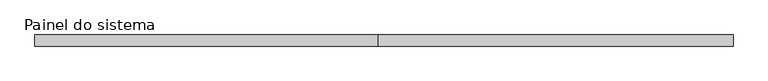
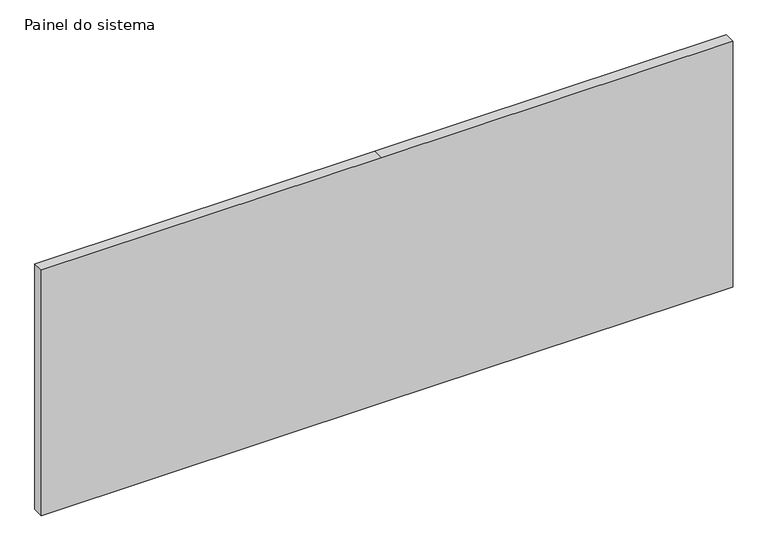
"""IFC4 building model written with IfcOpenShell, lengths in millimetres: plate geometry, Painel do sistema : Envidraçado."""

import ifcopenshell
import ifcopenshell.guid

model = None  # the IFC model being written
_history = None  # IfcOwnerHistory: only IFC2X3 demands one
_inside = {}  # id of a spatial element -> (the spatial element, [elements in it])
_under = {}  # id of a project, library or spatial element -> (it, [spatial elements below it])
_declared = {}  # id of a project -> (the project, [libraries it declares])
_typed = {}  # id of a type object -> (the type object, [elements of that type])
_made_of = {}  # id of a material, layer set ... -> (it, [elements and type objects made of it])


def new_model(schema):
    """Start an empty IFC model of exactly this schema.

    Asked for "IFC4X3", IfcOpenShell would pick the latest addendum, in which some entities
    have other attributes; the version numbers below select the first issue.
    IFC2X3 requires an IfcOwnerHistory on every rooted entity: one is made here for all.
    """
    global model, _history
    if schema == "IFC4X3":
        model = ifcopenshell.file(schema_version=(4, 3, 0, 0))
    else:
        model = ifcopenshell.file(schema=schema)
    _inside.clear()
    _under.clear()
    _declared.clear()
    _typed.clear()
    _made_of.clear()
    _history = None
    if model.schema == "IFC2X3":
        org = make("IfcOrganization", Name="unknown")
        user = make(
            "IfcPersonAndOrganization",
            ThePerson=make("IfcPerson", FamilyName="unknown"),
            TheOrganization=org,
        )
        app = make(
            "IfcApplication",
            ApplicationDeveloper=org,
            Version="unknown",
            ApplicationFullName="unknown",
            ApplicationIdentifier="unknown",
        )
        _history = make(
            "IfcOwnerHistory",
            OwningUser=user,
            OwningApplication=app,
            ChangeAction="ADDED",
            CreationDate=0,
        )
    return model


def make(cls, **values):
    """One entity of the class cls with the attributes given. An attribute that is None is left unset."""
    return model.create_entity(
        cls, **{name: value for name, value in values.items() if value is not None}
    )


def rooted(cls, **values):
    """An entity with a GlobalId (a new one), such as an element, a storey or a relation."""
    return make(cls, GlobalId=ifcopenshell.guid.new(), OwnerHistory=_history, **values)


def si_unit(unit_type, name, prefix=None):
    """IfcSIUnit, for example si_unit("LENGTHUNIT", "METRE", prefix="MILLI")."""
    return make("IfcSIUnit", UnitType=unit_type, Prefix=prefix, Name=name)


def assignment(units):
    """IfcUnitAssignment: the units of a project."""
    return None if units is None else make("IfcUnitAssignment", Units=units)


def point(xyz):
    """IfcCartesianPoint."""
    return None if xyz is None else make("IfcCartesianPoint", Coordinates=xyz)


def direction(xyz):
    """IfcDirection."""
    return None if xyz is None else make("IfcDirection", DirectionRatios=xyz)


def frame(location, z_axis=None, x_axis=None):
    """IfcAxis2Placement3D, a coordinate frame: its origin and axes. An axis left out is left unset."""
    return make(
        "IfcAxis2Placement3D",
        Location=point(location),
        Axis=direction(z_axis),
        RefDirection=direction(x_axis),
    )


def origin():
    """The frame at (0, 0, 0) with its axes left unset."""
    return frame((0.0, 0.0, 0.0))


def place(relative_to, where):
    """IfcLocalPlacement: puts the frame where relative to a parent placement (None: the world)."""
    return make(
        "IfcLocalPlacement", PlacementRelTo=relative_to, RelativePlacement=where
    )


def context(
    kind, dimensions, precision=None, world=None, true_north=None, identifier=None
):
    """IfcGeometricRepresentationContext, for example the 3D "Model" context."""
    return make(
        "IfcGeometricRepresentationContext",
        ContextIdentifier=identifier,
        ContextType=kind,
        CoordinateSpaceDimension=dimensions,
        Precision=precision,
        WorldCoordinateSystem=world,
        TrueNorth=true_north,
    )


def project(units=None, contexts=None):
    """IfcProject with its units and contexts."""
    return rooted(
        "IfcProject",
        Name="project",
        RepresentationContexts=contexts,
        UnitsInContext=assignment(units),
    )


def spatial(cls, under=None, at=None, **own):
    """A site, building, storey or space (cls), placed at a placement, below another one or the project."""
    s = rooted(cls, ObjectPlacement=at, **own)
    if under is not None:
        _under.setdefault(under.id(), (under, []))[1].append(s)
    return s


def polyline(points):
    """IfcPolyline through the points."""
    return make("IfcPolyline", Points=[point(p) for p in points])


def outline(outer, holes=None, kind="AREA"):
    """IfcArbitraryClosedProfileDef: a profile drawn as a closed curve; with holes, ...WithVoids."""
    if holes is None:
        return make("IfcArbitraryClosedProfileDef", ProfileType=kind, OuterCurve=outer)
    return make(
        "IfcArbitraryProfileDefWithVoids",
        ProfileType=kind,
        OuterCurve=outer,
        InnerCurves=holes,
    )


def extrude(swept, where, along, depth):
    """IfcExtrudedAreaSolid: the profile swept, set in the frame where, extruded along a direction by depth."""
    return make(
        "IfcExtrudedAreaSolid",
        SweptArea=swept,
        Position=where,
        ExtrudedDirection=direction(along),
        Depth=depth,
    )


def shape(context_of_items, identifier, shape_type, items):
    """IfcShapeRepresentation: the items that make up one representation, for example the "Body"."""
    return make(
        "IfcShapeRepresentation",
        ContextOfItems=context_of_items,
        RepresentationIdentifier=identifier,
        RepresentationType=shape_type,
        Items=items,
    )


def source(mapping_origin, context_of_items, identifier, shape_type, items):
    """IfcRepresentationMap: a shape defined once, which mapped items show again and again."""
    return make(
        "IfcRepresentationMap",
        MappingOrigin=mapping_origin,
        MappedRepresentation=shape(context_of_items, identifier, shape_type, items),
    )


def transform(
    local_origin,
    x_axis=None,
    y_axis=None,
    z_axis=None,
    scale=None,
    scale2=None,
    scale3=None,
    uniform=True,
):
    """IfcCartesianTransformationOperator3D, or its non-uniform kind. x_axis, y_axis, z_axis: its Axis1, 2, 3."""
    if uniform:
        return make(
            "IfcCartesianTransformationOperator3D",
            Axis1=direction(x_axis),
            Axis2=direction(y_axis),
            LocalOrigin=point(local_origin),
            Scale=scale,
            Axis3=direction(z_axis),
        )
    return make(
        "IfcCartesianTransformationOperator3DnonUniform",
        Axis1=direction(x_axis),
        Axis2=direction(y_axis),
        LocalOrigin=point(local_origin),
        Scale=scale,
        Axis3=direction(z_axis),
        Scale2=scale2,
        Scale3=scale3,
    )


def mapped(mapping_source, mapping_target):
    """IfcMappedItem: shows the shape of a source again, moved by a transform."""
    return make(
        "IfcMappedItem", MappingSource=mapping_source, MappingTarget=mapping_target
    )


def made_of(thing, what):
    """Note that an element or type object is made of a material, layer set ...; save() writes the relation."""
    if what is not None:
        _made_of.setdefault(what.id(), (what, []))[1].append(thing)
    return thing


def element(
    cls,
    number,
    at=None,
    inside=None,
    cuts=None,
    type_object=None,
    material=None,
    context=None,
    identifier="Body",
    shape_type=None,
    held_by="IfcProductDefinitionShape",
    body=None,
    shapes=None,
    **own,
):
    """One element of the class cls, such as IfcWall. Its Tag is "e" and its number.

    at: its placement. inside: the storey or other place that contains it. cuts: it is an
    opening in that element (IfcRelVoidsElement). A single representation is given by context,
    identifier, shape_type and body (its items); several are given by shapes. held_by: the class
    of the entity that holds the representations. save() writes the other relations.
    """
    e = rooted(cls, Tag="e%d" % number, ObjectPlacement=at, **own)
    if body is not None:
        shapes = [shape(context, identifier, shape_type, body)]
    if shapes is not None:
        e.Representation = make(held_by, Representations=shapes)
    if inside is not None:
        _inside.setdefault(inside.id(), (inside, []))[1].append(e)
    if cuts is not None:
        rooted(
            "IfcRelVoidsElement", RelatingBuildingElement=cuts, RelatedOpeningElement=e
        )
    if type_object is not None:
        _typed.setdefault(type_object.id(), (type_object, []))[1].append(e)
    return made_of(e, material)


def aggregate(whole, parts):
    """IfcRelAggregates: a whole, such as a stair, and the parts it consists of."""
    return rooted("IfcRelAggregates", RelatingObject=whole, RelatedObjects=parts)


def save(model, path):
    """Write the relations noted so far, then the file.

    IfcRelAggregates (storeys below a building ...), IfcRelContainedInSpatialStructure (elements
    in a storey), IfcRelDefinesByType, IfcRelAssociatesMaterial and IfcRelDeclares: one each for
    every whole, place, type object, material and project.
    """
    for whole, parts in _under.values():
        aggregate(whole, parts)
    for where, things in _inside.values():
        rooted(
            "IfcRelContainedInSpatialStructure",
            RelatedElements=things,
            RelatingStructure=where,
        )
    for kind, things in _typed.values():
        rooted("IfcRelDefinesByType", RelatedObjects=things, RelatingType=kind)
    for what, things in _made_of.values():
        rooted("IfcRelAssociatesMaterial", RelatedObjects=things, RelatingMaterial=what)
    for by, libraries in _declared.values():
        rooted("IfcRelDeclares", RelatingContext=by, RelatedDefinitions=libraries)
    model.write(path)


def painel_do_sistema_b434e0fb(model_context):
    return source(origin(), model_context, "Body", "SweptSolid", [
        extrude(outline(polyline([(0.0, -785.3166667), (0.0, -12.4999998), (0.0, 785.3166667), (590.0, 785.3166667), (590.0, -12.4999998), (590.0, -785.3166667), (0.0, -785.3166667)])), frame((0.0, -49.5, 0.0), z_axis=(0.0, 1.0, 0.0), x_axis=(0.0, 0.0, 1.0)), (0.0, 0.0, 1.0), 25.0),
    ])


if __name__ == "__main__":
    model = new_model("IFC4")
    model_context = context("Model", 3, world=origin())
    ifc_project = project(units=[si_unit("LENGTHUNIT", "METRE", prefix="MILLI")], contexts=[model_context])
    site = spatial("IfcSite", under=ifc_project)
    building = spatial("IfcBuilding", under=site)
    placement = place(None, origin())
    painel_do_sistema_shape = painel_do_sistema_b434e0fb(model_context)
    element("IfcPlate", 1, ObjectType="Painel do sistema : Envidraçado", at=placement, inside=building, context=model_context, shape_type="MappedRepresentation", body=[
        mapped(painel_do_sistema_shape, transform((0.0, 0.0, 0.0), x_axis=(1.0, 0.0, 0.0), y_axis=(0.0, 1.0, 0.0), z_axis=(0.0, 0.0, 1.0))),
    ])
    save(model, "model.ifc")

# Revit data of these elements
# Type "Painel do sistema : Envidraçado"
#   Construction Type Id = "GSP4R"
#   Analytic Construction = "Vidraça única Pilkington 1/8 pol"
#   Visual Light Transmittance = 0.9
#   Solar Heat Gain Coefficient = 0.86
#   Heat Transfer Coefficient (U) = 6.7069 W/(m²·K)
# Element 1 (IfcPlate, "Painel do sistema : Envidraçado")
#   Materials on its faces: ".VIDRO GENÉRICO"
# Materials
#   ".VIDRO GENÉRICO": class ".CC_VIDRO", colour RGB 0 128 192, transparency 0.9, Description = "Vidro comum", Cost = 0
